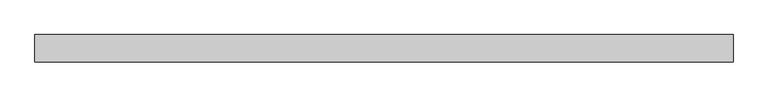
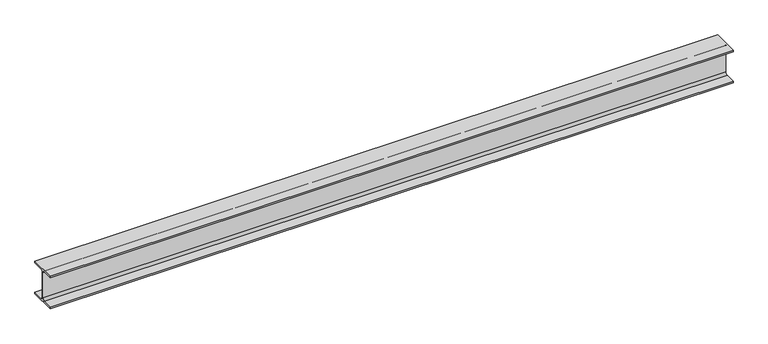
"""IFC4 building model written with IfcOpenShell, lengths in millimetres: beam geometry, 0912_Steel Framing_H-KSD3502 : H_SB_AR_S02_H-194x150x6x9_Platform."""

from ifc_helpers import new_model, si_unit, point, frame, frame_2d, origin, place, context, project, spatial, polyline, circle_curve, trimmed, segment, composite_curve, outline, extrude, source, transform, mapped, element, save


def beam_ff5aae68(model_context):
    return source(origin(), model_context, "Body", "SweptSolid", [
        extrude(outline(composite_curve([segment(polyline([(75.0, -88.0), (75.0, -97.0), (-75.0, -97.0), (-75.0, -88.0), (-16.0, -88.0)]), True, "CONTINUOUS"), segment(trimmed(circle_curve(frame_2d((-16.0, -75.0)), 13.0), [point((-16.0, -88.0))], [point((-3.0, -75.0))], True, "CARTESIAN"), True, "CONTINUOUS"), segment(polyline([(-3.0, -75.0), (-3.0, 75.0)]), True, "CONTINUOUS"), segment(trimmed(circle_curve(frame_2d((-16.0, 75.0)), 13.0), [point((-3.0, 75.0))], [point((-16.0, 88.0))], True, "CARTESIAN"), True, "CONTINUOUS"), segment(polyline([(-16.0, 88.0), (-75.0, 88.0), (-75.0, 97.0), (75.0, 97.0), (75.0, 88.0), (16.0, 88.0)]), True, "CONTINUOUS"), segment(trimmed(circle_curve(frame_2d((16.0, 75.0)), 13.0), [point((16.0, 88.0))], [point((3.0, 75.0))], True, "CARTESIAN"), True, "CONTINUOUS"), segment(polyline([(3.0, 75.0), (3.0, -75.0)]), True, "CONTINUOUS"), segment(trimmed(circle_curve(frame_2d((16.0, -75.0)), 13.0), [point((3.0, -75.0))], [point((16.0, -88.0))], True, "CARTESIAN"), True, "CONTINUOUS"), segment(polyline([(16.0, -88.0), (75.0, -88.0)]), True, "CONTINUOUS")], self_intersect=False)), frame((-1904.7357851, 0.0, 0.0), z_axis=(1.0, 0.0, 0.0), x_axis=(0.0, 1.0, 0.0)), (0.0, 0.0, 1.0), 3840.2404002),
    ])


if __name__ == "__main__":
    model = new_model("IFC4")
    model_context = context("Model", 3, world=origin())
    ifc_project = project(units=[si_unit("LENGTHUNIT", "METRE", prefix="MILLI")], contexts=[model_context])
    site = spatial("IfcSite", under=ifc_project)
    building = spatial("IfcBuilding", under=site)
    placement = place(None, origin())
    beam_shape = beam_ff5aae68(model_context)
    element("IfcBeam", 1, ObjectType="0912_Steel Framing_H-KSD3502 : H_SB_AR_S02_H-194x150x6x9_Platform", at=placement, inside=building, context=model_context, shape_type="MappedRepresentation", body=[
        mapped(beam_shape, transform((0.0, 0.0, 0.0), x_axis=(1.0, 0.0, 0.0), y_axis=(0.0, 1.0, 0.0), z_axis=(0.0, 0.0, 1.0))),
    ])
    save(model, "model.ifc")

# Revit data of these elements
# Type "0912_Steel Framing_H-KSD3502 : H_SB_AR_S02_H-194x150x6x9_Platform"
#   H_Q'ty Cal Type Tag = "SB-Q2"
#   H_WM Code_1 = "S01AA073-00001 |  | TON | Main Steel Structure Fabrication Work | Shelter/Building | Medium Steel - Standard |  |  |  |  |  |  | Material: (   ) | (90)KG/M>Weight≥(30)KG/M | S01AA073-00001 Main Steel Structure Fabrication Work Shelter/Building Medium Steel - Standard         | - Material: ( ASTM A36 )\n- (90)KG/M>Weight≥(30)KG/M"
#   H_WM Code_2 = "S03AA083-00001 |  | TON | Main Steel Structure Erection Work | Shelter/Building | Medium Steel |  |  |  |  |  |  | Material: (   ) | S03AA083-00001 Main Steel Structure Erection Work Shelter/Building Medium Steel         | - Material: ( ASTM A36 )"
#   H_WM Code_3 = "S01AA009-00001 |  | TON | Main Steel Structure Fabrication Work | Shelter/Building | Plates - Gusset, Stiffener, ETC | Material: (   ) | S01AA009-00001 Main Steel Structure Fabrication Work Shelter/Building Plates - Gusset, Stiffener, ETC         |"
#   H_WM Code_4 = "S41AA051-00001 |  | M2 | Steel Structure Paint Work | Shelter/Building | for Non-Fireproofed Steel Surface |  |  |  |  |  |  | Material: (   ) | S41AA051-00001 Steel Structure Paint Work Shelter/Building for Non-Fireproofed Steel Surface         |"
#   Width = 15.0 cm
#   Web Thickness = 0.6 cm
#   Web Fillet = 1.3 cm
#   Warping Constant = 43316.0 cm⁶
#   W = 0
#   Torsional Moment of Inertia = 8.622 cm⁴
#   Section Area = 39.01 cm²
#   Plastic Modulus weak axis = 104.0 cm³
#   Plastic Modulus strong axis = 309.0 cm³
#   Perimeter = 0.95 m²/m
#   Nominal Weight = 30.60 kgf/m
#   Moment of Inertia weak axis = 507.00 cm⁴
#   Moment of Inertia strong axis = 2690.00 cm⁴
#   Height = 19.4 cm
#   Flange Thickness = 0.9 cm
#   Elastic Modulus weak axis = 67.6 cm³
#   Elastic Modulus strong axis = 277.0 cm³
#   Centroid Vertical = 9.7 cm
#   Centroid Horizontal = 7.5 cm
#   Ix = 26900000
#   Length [instance default] = 1524 mm
#   Zx = 309000
#   b = 150 mm
#   h = 194 mm
#   r = 13 mm
#   s = 6 mm
#   t = 9 mm
#   A = 0.003901 m²
#   Structural Material [instance default] = Steel, 45-345
#   Assembly Code = ""
# Element 1 (IfcBeam, "0912_Steel Framing_H-KSD3502 : H_SB_AR_S02_H-194x150x6x9_Platform")
#   Materials on its faces: "Steel, 45-345"
# Materials
#   "Steel, 45-345": class "Metal", colour RGB 189 187 185, transparency 0, Description = "Steel 345 MPa", Cost = 0
